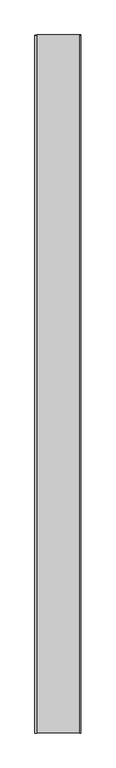
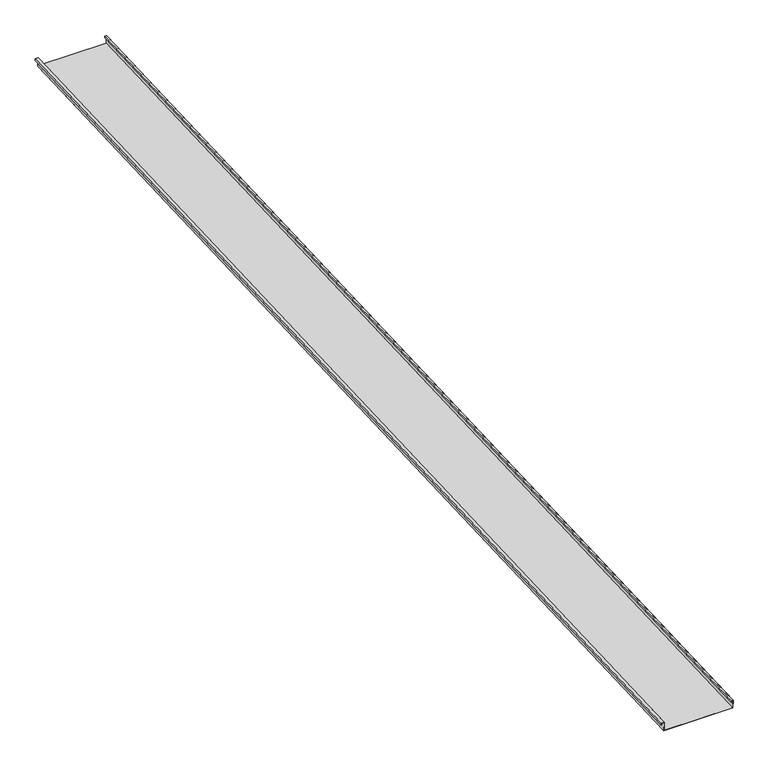
"""IFC4 building model written with IfcOpenShell, lengths in millimetres: proxy geometry, Generic Models 2:Generic Models 2:310765:Generic Models 2:310765 : Generic Models 2:Generic Models 2:310765:122 : Generic Models 2:Generic Models 2:310765:Generic Models 2:310765 : Generic Models 2:Generic Models 2:310765:300385."""

from ifc_helpers import new_model, si_unit, frame, origin, place, context, project, spatial, polyline, outline, extrude, source, transform, mapped, element, save


def generic_models_2677ad0b(model_context):
    return source(origin(), model_context, "Body", "SweptSolid", [
        extrude(outline(polyline([(1.5875, 0.0), (1.5875, 50.8), (407.9875, 50.8), (407.9875, 1.5875), (396.875, 1.5875), (396.875, 11.1125), (398.4625, 11.1125), (398.4625, 3.175), (406.4, 3.175), (406.4, 49.2125), (3.175, 49.2125), (3.175, -1.5874999), (-14.2875, -1.5874999), (-14.2875, 9.525), (-12.7, 9.525), (-12.7, 0.0), (1.5875, 0.0)])), frame((664618.1096405, -581354.4345603, 3902.6697972), z_axis=(0.0, 0.9991330730923568, 0.041630544712067834), x_axis=(1.0, 0.0, 0.0)), (0.0, 0.0, 1.0), 6400.8),
    ])


if __name__ == "__main__":
    model = new_model("IFC4")
    model_context = context("Model", 3, world=origin())
    ifc_project = project(units=[si_unit("LENGTHUNIT", "METRE", prefix="MILLI")], contexts=[model_context])
    site = spatial("IfcSite", under=ifc_project)
    building = spatial("IfcBuilding", under=site)
    placement = place(None, origin())
    generic_models_shape = generic_models_2677ad0b(model_context)
    element("IfcBuildingElementProxy", 1, Name="Generic Models 2:Generic Models 2:310765:Generic Models 2:310765 : Generic Models 2:Generic Models 2:310765:122 : Generic Models 2:Generic Models 2:310765:Generic Models 2:310765 : Generic Models 2:Generic Models 2:310765:300385", ObjectType="Generic Models 2:Generic Models 2:310765:Generic Models 2:310765 : Generic Models 2:Generic Models 2:310765:122 : Generic Models 2:Generic Models 2:310765:Generic Models 2:310765 : Generic Models 2:Generic Models 2:310765:300385", at=placement, inside=building, context=model_context, shape_type="MappedRepresentation", body=[
        mapped(generic_models_shape, transform((0.0, 0.0, 0.0), x_axis=(1.0, 0.0, 0.0), y_axis=(0.0, 1.0, 0.0), z_axis=(0.0, 0.0, 1.0))),
    ])
    save(model, "model.ifc")

# Revit data of these elements
# Type "Generic Models 2:Generic Models 2:310765:Generic Models 2:310765 : Generic Models 2:Generic Models 2:310765:122 : Generic Models 2:Generic Models 2:310765:Generic Models 2:310765 : Generic Models 2:Generic Models 2:310765:300385"
#   NameOverride = "Generic Models 2:Generic Models 2:310765:Generic Models 2:310765 : Generic Models 2:Generic Models 2:310765:300385"
#   ObjectTypeOverride = "Generic Models 2:310765 : Generic Models 2:Generic Models 2:310765"
#   Reference = "Generic Models 2"
#   Tag = "300385"
# Element 1 (IfcBuildingElementProxy, "Generic Models 2:Generic Models 2:310765:Generic Models 2:310765 : Generic Models 2:Generic Models 2:310765:122 : Generic Models 2:Generic Models 2:310765:Generic Models 2:310765 : Generic Models 2:Generic Models 2:310765:300385")
#   Materials on its faces: "THERMAL BROKEN ALUMINUM STOREFRONT FOR POLYCARBONATE"
# Materials
#   "THERMAL BROKEN ALUMINUM STOREFRONT FOR POLYCARBONATE": class "Unassigned", colour RGB 244 244 244, transparency 0, Keynote = "M07611300.01", Cost = 0
